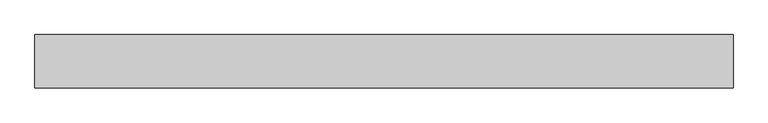
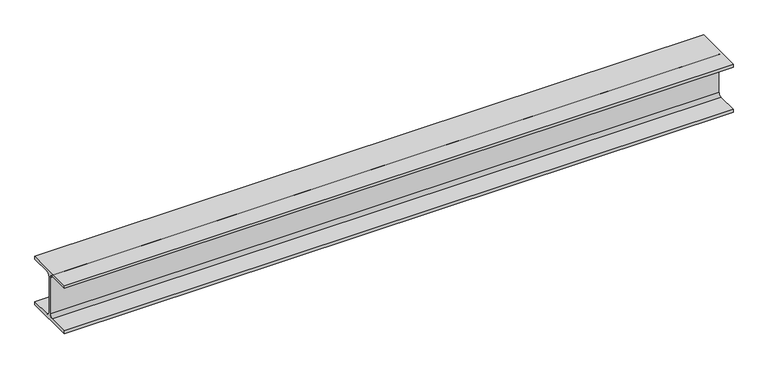
"""IFC4 building model written with IfcOpenShell, lengths in millimetres: beam geometry, 0912_Steel Framing_H-KSD3502 : H_SB_ASB_H-200x200x8x12."""

import ifcopenshell
import ifcopenshell.guid

model = None  # the IFC model being written
_history = None  # IfcOwnerHistory: only IFC2X3 demands one
_inside = {}  # id of a spatial element -> (the spatial element, [elements in it])
_under = {}  # id of a project, library or spatial element -> (it, [spatial elements below it])
_declared = {}  # id of a project -> (the project, [libraries it declares])
_typed = {}  # id of a type object -> (the type object, [elements of that type])
_made_of = {}  # id of a material, layer set ... -> (it, [elements and type objects made of it])


def new_model(schema):
    """Start an empty IFC model of exactly this schema.

    Asked for "IFC4X3", IfcOpenShell would pick the latest addendum, in which some entities
    have other attributes; the version numbers below select the first issue.
    IFC2X3 requires an IfcOwnerHistory on every rooted entity: one is made here for all.
    """
    global model, _history
    if schema == "IFC4X3":
        model = ifcopenshell.file(schema_version=(4, 3, 0, 0))
    else:
        model = ifcopenshell.file(schema=schema)
    _inside.clear()
    _under.clear()
    _declared.clear()
    _typed.clear()
    _made_of.clear()
    _history = None
    if model.schema == "IFC2X3":
        org = make("IfcOrganization", Name="unknown")
        user = make(
            "IfcPersonAndOrganization",
            ThePerson=make("IfcPerson", FamilyName="unknown"),
            TheOrganization=org,
        )
        app = make(
            "IfcApplication",
            ApplicationDeveloper=org,
            Version="unknown",
            ApplicationFullName="unknown",
            ApplicationIdentifier="unknown",
        )
        _history = make(
            "IfcOwnerHistory",
            OwningUser=user,
            OwningApplication=app,
            ChangeAction="ADDED",
            CreationDate=0,
        )
    return model


def make(cls, **values):
    """One entity of the class cls with the attributes given. An attribute that is None is left unset."""
    return model.create_entity(
        cls, **{name: value for name, value in values.items() if value is not None}
    )


def rooted(cls, **values):
    """An entity with a GlobalId (a new one), such as an element, a storey or a relation."""
    return make(cls, GlobalId=ifcopenshell.guid.new(), OwnerHistory=_history, **values)


def si_unit(unit_type, name, prefix=None):
    """IfcSIUnit, for example si_unit("LENGTHUNIT", "METRE", prefix="MILLI")."""
    return make("IfcSIUnit", UnitType=unit_type, Prefix=prefix, Name=name)


def assignment(units):
    """IfcUnitAssignment: the units of a project."""
    return None if units is None else make("IfcUnitAssignment", Units=units)


def point(xyz):
    """IfcCartesianPoint."""
    return None if xyz is None else make("IfcCartesianPoint", Coordinates=xyz)


def direction(xyz):
    """IfcDirection."""
    return None if xyz is None else make("IfcDirection", DirectionRatios=xyz)


def frame(location, z_axis=None, x_axis=None):
    """IfcAxis2Placement3D, a coordinate frame: its origin and axes. An axis left out is left unset."""
    return make(
        "IfcAxis2Placement3D",
        Location=point(location),
        Axis=direction(z_axis),
        RefDirection=direction(x_axis),
    )


def frame_2d(location, x_axis=None):
    """IfcAxis2Placement2D, a coordinate frame in the plane: its origin and x axis."""
    return make(
        "IfcAxis2Placement2D", Location=point(location), RefDirection=direction(x_axis)
    )


def origin():
    """The frame at (0, 0, 0) with its axes left unset."""
    return frame((0.0, 0.0, 0.0))


def place(relative_to, where):
    """IfcLocalPlacement: puts the frame where relative to a parent placement (None: the world)."""
    return make(
        "IfcLocalPlacement", PlacementRelTo=relative_to, RelativePlacement=where
    )


def context(
    kind, dimensions, precision=None, world=None, true_north=None, identifier=None
):
    """IfcGeometricRepresentationContext, for example the 3D "Model" context."""
    return make(
        "IfcGeometricRepresentationContext",
        ContextIdentifier=identifier,
        ContextType=kind,
        CoordinateSpaceDimension=dimensions,
        Precision=precision,
        WorldCoordinateSystem=world,
        TrueNorth=true_north,
    )


def project(units=None, contexts=None):
    """IfcProject with its units and contexts."""
    return rooted(
        "IfcProject",
        Name="project",
        RepresentationContexts=contexts,
        UnitsInContext=assignment(units),
    )


def spatial(cls, under=None, at=None, **own):
    """A site, building, storey or space (cls), placed at a placement, below another one or the project."""
    s = rooted(cls, ObjectPlacement=at, **own)
    if under is not None:
        _under.setdefault(under.id(), (under, []))[1].append(s)
    return s


def polyline(points):
    """IfcPolyline through the points."""
    return make("IfcPolyline", Points=[point(p) for p in points])


def circle_curve(where, radius):
    """IfcCircle in the frame where."""
    return make("IfcCircle", Position=where, Radius=radius)


def trimmed(basis, trim1, trim2, sense, master):
    """IfcTrimmedCurve: the piece of a basis curve between two trims."""
    return make(
        "IfcTrimmedCurve",
        BasisCurve=basis,
        Trim1=trim1,
        Trim2=trim2,
        SenseAgreement=sense,
        MasterRepresentation=master,
    )


def segment(curve, same_sense, transition):
    """IfcCompositeCurveSegment."""
    return make(
        "IfcCompositeCurveSegment",
        Transition=transition,
        SameSense=same_sense,
        ParentCurve=curve,
    )


def composite_curve(segments, self_intersect=None):
    """IfcCompositeCurve: segments joined end to end."""
    return make("IfcCompositeCurve", Segments=segments, SelfIntersect=self_intersect)


def outline(outer, holes=None, kind="AREA"):
    """IfcArbitraryClosedProfileDef: a profile drawn as a closed curve; with holes, ...WithVoids."""
    if holes is None:
        return make("IfcArbitraryClosedProfileDef", ProfileType=kind, OuterCurve=outer)
    return make(
        "IfcArbitraryProfileDefWithVoids",
        ProfileType=kind,
        OuterCurve=outer,
        InnerCurves=holes,
    )


def extrude(swept, where, along, depth):
    """IfcExtrudedAreaSolid: the profile swept, set in the frame where, extruded along a direction by depth."""
    return make(
        "IfcExtrudedAreaSolid",
        SweptArea=swept,
        Position=where,
        ExtrudedDirection=direction(along),
        Depth=depth,
    )


def shape(context_of_items, identifier, shape_type, items):
    """IfcShapeRepresentation: the items that make up one representation, for example the "Body"."""
    return make(
        "IfcShapeRepresentation",
        ContextOfItems=context_of_items,
        RepresentationIdentifier=identifier,
        RepresentationType=shape_type,
        Items=items,
    )


def source(mapping_origin, context_of_items, identifier, shape_type, items):
    """IfcRepresentationMap: a shape defined once, which mapped items show again and again."""
    return make(
        "IfcRepresentationMap",
        MappingOrigin=mapping_origin,
        MappedRepresentation=shape(context_of_items, identifier, shape_type, items),
    )


def transform(
    local_origin,
    x_axis=None,
    y_axis=None,
    z_axis=None,
    scale=None,
    scale2=None,
    scale3=None,
    uniform=True,
):
    """IfcCartesianTransformationOperator3D, or its non-uniform kind. x_axis, y_axis, z_axis: its Axis1, 2, 3."""
    if uniform:
        return make(
            "IfcCartesianTransformationOperator3D",
            Axis1=direction(x_axis),
            Axis2=direction(y_axis),
            LocalOrigin=point(local_origin),
            Scale=scale,
            Axis3=direction(z_axis),
        )
    return make(
        "IfcCartesianTransformationOperator3DnonUniform",
        Axis1=direction(x_axis),
        Axis2=direction(y_axis),
        LocalOrigin=point(local_origin),
        Scale=scale,
        Axis3=direction(z_axis),
        Scale2=scale2,
        Scale3=scale3,
    )


def mapped(mapping_source, mapping_target):
    """IfcMappedItem: shows the shape of a source again, moved by a transform."""
    return make(
        "IfcMappedItem", MappingSource=mapping_source, MappingTarget=mapping_target
    )


def made_of(thing, what):
    """Note that an element or type object is made of a material, layer set ...; save() writes the relation."""
    if what is not None:
        _made_of.setdefault(what.id(), (what, []))[1].append(thing)
    return thing


def element(
    cls,
    number,
    at=None,
    inside=None,
    cuts=None,
    type_object=None,
    material=None,
    context=None,
    identifier="Body",
    shape_type=None,
    held_by="IfcProductDefinitionShape",
    body=None,
    shapes=None,
    **own,
):
    """One element of the class cls, such as IfcWall. Its Tag is "e" and its number.

    at: its placement. inside: the storey or other place that contains it. cuts: it is an
    opening in that element (IfcRelVoidsElement). A single representation is given by context,
    identifier, shape_type and body (its items); several are given by shapes. held_by: the class
    of the entity that holds the representations. save() writes the other relations.
    """
    e = rooted(cls, Tag="e%d" % number, ObjectPlacement=at, **own)
    if body is not None:
        shapes = [shape(context, identifier, shape_type, body)]
    if shapes is not None:
        e.Representation = make(held_by, Representations=shapes)
    if inside is not None:
        _inside.setdefault(inside.id(), (inside, []))[1].append(e)
    if cuts is not None:
        rooted(
            "IfcRelVoidsElement", RelatingBuildingElement=cuts, RelatedOpeningElement=e
        )
    if type_object is not None:
        _typed.setdefault(type_object.id(), (type_object, []))[1].append(e)
    return made_of(e, material)


def aggregate(whole, parts):
    """IfcRelAggregates: a whole, such as a stair, and the parts it consists of."""
    return rooted("IfcRelAggregates", RelatingObject=whole, RelatedObjects=parts)


def save(model, path):
    """Write the relations noted so far, then the file.

    IfcRelAggregates (storeys below a building ...), IfcRelContainedInSpatialStructure (elements
    in a storey), IfcRelDefinesByType, IfcRelAssociatesMaterial and IfcRelDeclares: one each for
    every whole, place, type object, material and project.
    """
    for whole, parts in _under.values():
        aggregate(whole, parts)
    for where, things in _inside.values():
        rooted(
            "IfcRelContainedInSpatialStructure",
            RelatedElements=things,
            RelatingStructure=where,
        )
    for kind, things in _typed.values():
        rooted("IfcRelDefinesByType", RelatedObjects=things, RelatingType=kind)
    for what, things in _made_of.values():
        rooted("IfcRelAssociatesMaterial", RelatedObjects=things, RelatingMaterial=what)
    for by, libraries in _declared.values():
        rooted("IfcRelDeclares", RelatingContext=by, RelatedDefinitions=libraries)
    model.write(path)


def beam_192a384f(model_context):
    return source(origin(), model_context, "Body", "SweptSolid", [
        extrude(outline(composite_curve([segment(polyline([(100.0, -88.0), (100.0, -100.0), (-100.0, -100.0), (-100.0, -88.0), (-17.0, -88.0)]), True, "CONTINUOUS"), segment(trimmed(circle_curve(frame_2d((-17.0, -75.0)), 13.0), [point((-17.0, -88.0))], [point((-4.0, -75.0))], True, "CARTESIAN"), True, "CONTINUOUS"), segment(polyline([(-4.0, -75.0), (-4.0, 75.0)]), True, "CONTINUOUS"), segment(trimmed(circle_curve(frame_2d((-17.0, 75.0)), 13.0), [point((-4.0, 75.0))], [point((-17.0, 88.0))], True, "CARTESIAN"), True, "CONTINUOUS"), segment(polyline([(-17.0, 88.0), (-100.0, 88.0), (-100.0, 100.0), (100.0, 100.0), (100.0, 88.0), (17.0, 88.0)]), True, "CONTINUOUS"), segment(trimmed(circle_curve(frame_2d((17.0, 75.0)), 13.0), [point((17.0, 88.0))], [point((4.0, 75.0))], True, "CARTESIAN"), True, "CONTINUOUS"), segment(polyline([(4.0, 75.0), (4.0, -75.0)]), True, "CONTINUOUS"), segment(trimmed(circle_curve(frame_2d((17.0, -75.0)), 13.0), [point((4.0, -75.0))], [point((17.0, -88.0))], True, "CARTESIAN"), True, "CONTINUOUS"), segment(polyline([(17.0, -88.0), (100.0, -88.0)]), True, "CONTINUOUS")], self_intersect=False)), frame((-1295.3889401, 0.0, 0.0), z_axis=(1.0, 0.0, 0.0), x_axis=(0.0, 1.0, 0.0)), (0.0, 0.0, 1.0), 2624.3471578),
    ])


if __name__ == "__main__":
    model = new_model("IFC4")
    model_context = context("Model", 3, world=origin())
    ifc_project = project(units=[si_unit("LENGTHUNIT", "METRE", prefix="MILLI")], contexts=[model_context])
    site = spatial("IfcSite", under=ifc_project)
    building = spatial("IfcBuilding", under=site)
    placement = place(None, origin())
    beam_shape = beam_192a384f(model_context)
    element("IfcBeam", 1, ObjectType="0912_Steel Framing_H-KSD3502 : H_SB_ASB_H-200x200x8x12", at=placement, inside=building, context=model_context, shape_type="MappedRepresentation", body=[
        mapped(beam_shape, transform((0.0, 0.0, 0.0), x_axis=(1.0, 0.0, 0.0), y_axis=(0.0, 1.0, 0.0), z_axis=(0.0, 0.0, 1.0))),
    ])
    save(model, "model.ifc")

# Revit data of these elements
# Type "0912_Steel Framing_H-KSD3502 : H_SB_ASB_H-200x200x8x12"
#   H_WM Code_1 = "S01AA002-00001 | Main Steel Structure Fabrication Work | Shelter/Building | Medium Steel - Standard (90KG/M>Weight≥30KG/M) | Material: (   )"
#   H_WM Code_2 = "S03AA028-00001 | Main Steel Structure Erection Work | Shelter/Building | Medium Steel (90KG/M>Weight≥30KG/M) | Material: (   )"
#   H_WM Code_3 = "S01AA010-00001 | Main Steel Structure Fabrication Work | Shelter/Building | Steel Painting/Coating | for Non-Fireproofed Steel Surface, Surface Preparation, Primer, Second & Final Coat | Material: (   )"
#   H_Q'ty Cal Type Tag = "SB-Q2"
#   Width = 20.0 cm
#   Web Thickness = 0.8 cm
#   Web Fillet = 1.3 cm
#   Warping Constant = 141000.0 cm⁶
#   W = 0
#   Torsional Moment of Inertia = 26.2485 cm⁴
#   Section Area = 63.53 cm²
#   Plastic Modulus weak axis = 244.0 cm³
#   Plastic Modulus strong axis = 525.0 cm³
#   Perimeter = 1.16 m²/m
#   Nominal Weight = 49.90 kgf/m
#   Moment of Inertia weak axis = 1600.00 cm⁴
#   Moment of Inertia strong axis = 4720.00 cm⁴
#   Height = 20.0 cm
#   Flange Thickness = 1.2 cm
#   Elastic Modulus weak axis = 160.0 cm³
#   Elastic Modulus strong axis = 472.0 cm³
#   Centroid Vertical = 10.0 cm
#   Centroid Horizontal = 10.0 cm
#   Ix = 47200000
#   Length [instance default] = 1.5240 m
#   Zx = 525000
#   b = 0.2000 m
#   h = 0.2000 m
#   r = 0.0130 m
#   s = 0.0080 m
#   t = 0.0120 m
#   A = 0.006353 m²
#   Structural Material [instance default] = Steel, 45-345
#   Assembly Code = ""
# Element 1 (IfcBeam, "0912_Steel Framing_H-KSD3502 : H_SB_ASB_H-200x200x8x12")
#   Structural Material = none
# Materials
#   "Steel, 45-345": class "Metal", colour RGB 189 187 185, transparency 0, Description = "Steel 345 MPa", Cost = 0
